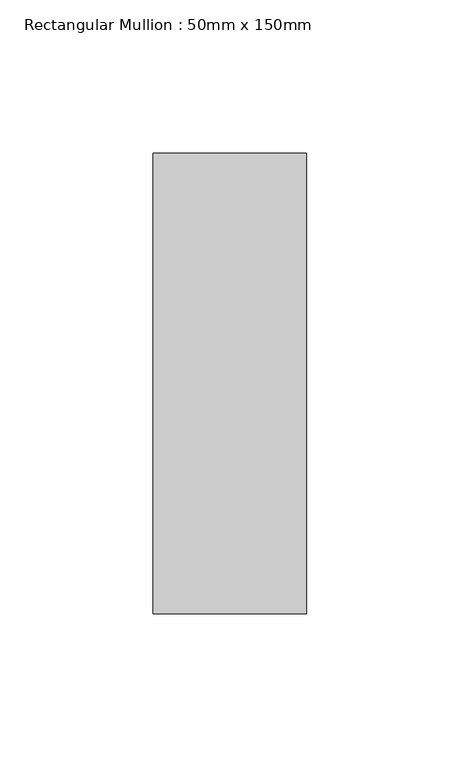
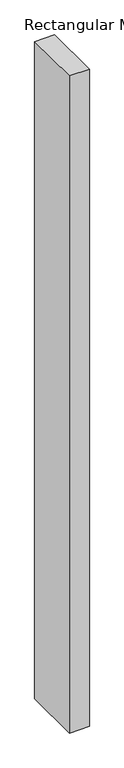
"""IFC4 building model written with IfcOpenShell, lengths in millimetres: member geometry, Rectangular Mullion : 50mm x 150mm."""

import ifcopenshell
import ifcopenshell.guid

model = None  # the IFC model being written
_history = None  # IfcOwnerHistory: only IFC2X3 demands one
_inside = {}  # id of a spatial element -> (the spatial element, [elements in it])
_under = {}  # id of a project, library or spatial element -> (it, [spatial elements below it])
_declared = {}  # id of a project -> (the project, [libraries it declares])
_typed = {}  # id of a type object -> (the type object, [elements of that type])
_made_of = {}  # id of a material, layer set ... -> (it, [elements and type objects made of it])


def new_model(schema):
    """Start an empty IFC model of exactly this schema.

    Asked for "IFC4X3", IfcOpenShell would pick the latest addendum, in which some entities
    have other attributes; the version numbers below select the first issue.
    IFC2X3 requires an IfcOwnerHistory on every rooted entity: one is made here for all.
    """
    global model, _history
    if schema == "IFC4X3":
        model = ifcopenshell.file(schema_version=(4, 3, 0, 0))
    else:
        model = ifcopenshell.file(schema=schema)
    _inside.clear()
    _under.clear()
    _declared.clear()
    _typed.clear()
    _made_of.clear()
    _history = None
    if model.schema == "IFC2X3":
        org = make("IfcOrganization", Name="unknown")
        user = make(
            "IfcPersonAndOrganization",
            ThePerson=make("IfcPerson", FamilyName="unknown"),
            TheOrganization=org,
        )
        app = make(
            "IfcApplication",
            ApplicationDeveloper=org,
            Version="unknown",
            ApplicationFullName="unknown",
            ApplicationIdentifier="unknown",
        )
        _history = make(
            "IfcOwnerHistory",
            OwningUser=user,
            OwningApplication=app,
            ChangeAction="ADDED",
            CreationDate=0,
        )
    return model


def make(cls, **values):
    """One entity of the class cls with the attributes given. An attribute that is None is left unset."""
    return model.create_entity(
        cls, **{name: value for name, value in values.items() if value is not None}
    )


def rooted(cls, **values):
    """An entity with a GlobalId (a new one), such as an element, a storey or a relation."""
    return make(cls, GlobalId=ifcopenshell.guid.new(), OwnerHistory=_history, **values)


def si_unit(unit_type, name, prefix=None):
    """IfcSIUnit, for example si_unit("LENGTHUNIT", "METRE", prefix="MILLI")."""
    return make("IfcSIUnit", UnitType=unit_type, Prefix=prefix, Name=name)


def assignment(units):
    """IfcUnitAssignment: the units of a project."""
    return None if units is None else make("IfcUnitAssignment", Units=units)


def point(xyz):
    """IfcCartesianPoint."""
    return None if xyz is None else make("IfcCartesianPoint", Coordinates=xyz)


def direction(xyz):
    """IfcDirection."""
    return None if xyz is None else make("IfcDirection", DirectionRatios=xyz)


def frame(location, z_axis=None, x_axis=None):
    """IfcAxis2Placement3D, a coordinate frame: its origin and axes. An axis left out is left unset."""
    return make(
        "IfcAxis2Placement3D",
        Location=point(location),
        Axis=direction(z_axis),
        RefDirection=direction(x_axis),
    )


def origin():
    """The frame at (0, 0, 0) with its axes left unset."""
    return frame((0.0, 0.0, 0.0))


def place(relative_to, where):
    """IfcLocalPlacement: puts the frame where relative to a parent placement (None: the world)."""
    return make(
        "IfcLocalPlacement", PlacementRelTo=relative_to, RelativePlacement=where
    )


def context(
    kind, dimensions, precision=None, world=None, true_north=None, identifier=None
):
    """IfcGeometricRepresentationContext, for example the 3D "Model" context."""
    return make(
        "IfcGeometricRepresentationContext",
        ContextIdentifier=identifier,
        ContextType=kind,
        CoordinateSpaceDimension=dimensions,
        Precision=precision,
        WorldCoordinateSystem=world,
        TrueNorth=true_north,
    )


def project(units=None, contexts=None):
    """IfcProject with its units and contexts."""
    return rooted(
        "IfcProject",
        Name="project",
        RepresentationContexts=contexts,
        UnitsInContext=assignment(units),
    )


def spatial(cls, under=None, at=None, **own):
    """A site, building, storey or space (cls), placed at a placement, below another one or the project."""
    s = rooted(cls, ObjectPlacement=at, **own)
    if under is not None:
        _under.setdefault(under.id(), (under, []))[1].append(s)
    return s


def polyline(points):
    """IfcPolyline through the points."""
    return make("IfcPolyline", Points=[point(p) for p in points])


def outline(outer, holes=None, kind="AREA"):
    """IfcArbitraryClosedProfileDef: a profile drawn as a closed curve; with holes, ...WithVoids."""
    if holes is None:
        return make("IfcArbitraryClosedProfileDef", ProfileType=kind, OuterCurve=outer)
    return make(
        "IfcArbitraryProfileDefWithVoids",
        ProfileType=kind,
        OuterCurve=outer,
        InnerCurves=holes,
    )


def extrude(swept, where, along, depth):
    """IfcExtrudedAreaSolid: the profile swept, set in the frame where, extruded along a direction by depth."""
    return make(
        "IfcExtrudedAreaSolid",
        SweptArea=swept,
        Position=where,
        ExtrudedDirection=direction(along),
        Depth=depth,
    )


def shape(context_of_items, identifier, shape_type, items):
    """IfcShapeRepresentation: the items that make up one representation, for example the "Body"."""
    return make(
        "IfcShapeRepresentation",
        ContextOfItems=context_of_items,
        RepresentationIdentifier=identifier,
        RepresentationType=shape_type,
        Items=items,
    )


def source(mapping_origin, context_of_items, identifier, shape_type, items):
    """IfcRepresentationMap: a shape defined once, which mapped items show again and again."""
    return make(
        "IfcRepresentationMap",
        MappingOrigin=mapping_origin,
        MappedRepresentation=shape(context_of_items, identifier, shape_type, items),
    )


def transform(
    local_origin,
    x_axis=None,
    y_axis=None,
    z_axis=None,
    scale=None,
    scale2=None,
    scale3=None,
    uniform=True,
):
    """IfcCartesianTransformationOperator3D, or its non-uniform kind. x_axis, y_axis, z_axis: its Axis1, 2, 3."""
    if uniform:
        return make(
            "IfcCartesianTransformationOperator3D",
            Axis1=direction(x_axis),
            Axis2=direction(y_axis),
            LocalOrigin=point(local_origin),
            Scale=scale,
            Axis3=direction(z_axis),
        )
    return make(
        "IfcCartesianTransformationOperator3DnonUniform",
        Axis1=direction(x_axis),
        Axis2=direction(y_axis),
        LocalOrigin=point(local_origin),
        Scale=scale,
        Axis3=direction(z_axis),
        Scale2=scale2,
        Scale3=scale3,
    )


def mapped(mapping_source, mapping_target):
    """IfcMappedItem: shows the shape of a source again, moved by a transform."""
    return make(
        "IfcMappedItem", MappingSource=mapping_source, MappingTarget=mapping_target
    )


def made_of(thing, what):
    """Note that an element or type object is made of a material, layer set ...; save() writes the relation."""
    if what is not None:
        _made_of.setdefault(what.id(), (what, []))[1].append(thing)
    return thing


def element(
    cls,
    number,
    at=None,
    inside=None,
    cuts=None,
    type_object=None,
    material=None,
    context=None,
    identifier="Body",
    shape_type=None,
    held_by="IfcProductDefinitionShape",
    body=None,
    shapes=None,
    **own,
):
    """One element of the class cls, such as IfcWall. Its Tag is "e" and its number.

    at: its placement. inside: the storey or other place that contains it. cuts: it is an
    opening in that element (IfcRelVoidsElement). A single representation is given by context,
    identifier, shape_type and body (its items); several are given by shapes. held_by: the class
    of the entity that holds the representations. save() writes the other relations.
    """
    e = rooted(cls, Tag="e%d" % number, ObjectPlacement=at, **own)
    if body is not None:
        shapes = [shape(context, identifier, shape_type, body)]
    if shapes is not None:
        e.Representation = make(held_by, Representations=shapes)
    if inside is not None:
        _inside.setdefault(inside.id(), (inside, []))[1].append(e)
    if cuts is not None:
        rooted(
            "IfcRelVoidsElement", RelatingBuildingElement=cuts, RelatedOpeningElement=e
        )
    if type_object is not None:
        _typed.setdefault(type_object.id(), (type_object, []))[1].append(e)
    return made_of(e, material)


def aggregate(whole, parts):
    """IfcRelAggregates: a whole, such as a stair, and the parts it consists of."""
    return rooted("IfcRelAggregates", RelatingObject=whole, RelatedObjects=parts)


def save(model, path):
    """Write the relations noted so far, then the file.

    IfcRelAggregates (storeys below a building ...), IfcRelContainedInSpatialStructure (elements
    in a storey), IfcRelDefinesByType, IfcRelAssociatesMaterial and IfcRelDeclares: one each for
    every whole, place, type object, material and project.
    """
    for whole, parts in _under.values():
        aggregate(whole, parts)
    for where, things in _inside.values():
        rooted(
            "IfcRelContainedInSpatialStructure",
            RelatedElements=things,
            RelatingStructure=where,
        )
    for kind, things in _typed.values():
        rooted("IfcRelDefinesByType", RelatedObjects=things, RelatingType=kind)
    for what, things in _made_of.values():
        rooted("IfcRelAssociatesMaterial", RelatedObjects=things, RelatingMaterial=what)
    for by, libraries in _declared.values():
        rooted("IfcRelDeclares", RelatingContext=by, RelatedDefinitions=libraries)
    model.write(path)


def rectangular_mullion_50mm_x_150mm_0deb6731(model_context):
    return source(origin(), model_context, "Body", "SweptSolid", [
        extrude(outline(polyline([(0.0, 75.0), (0.0, -75.0), (-50.0, -75.0), (-50.0, 75.0), (0.0, 75.0)])), frame((0.0, 0.0, -1736.2355347), z_axis=(0.0, 0.0, 1.0), x_axis=(1.0, 0.0, 0.0)), (0.0, 0.0, 1.0), 1736.2355347),
    ])


if __name__ == "__main__":
    model = new_model("IFC4")
    model_context = context("Model", 3, world=origin())
    ifc_project = project(units=[si_unit("LENGTHUNIT", "METRE", prefix="MILLI")], contexts=[model_context])
    site = spatial("IfcSite", under=ifc_project)
    building = spatial("IfcBuilding", under=site)
    placement = place(None, origin())
    rectangular_mullion_50mm_x_150mm_shape = rectangular_mullion_50mm_x_150mm_0deb6731(model_context)
    element("IfcMember", 1, ObjectType="Rectangular Mullion : 50mm x 150mm", at=placement, inside=building, context=model_context, shape_type="MappedRepresentation", body=[
        mapped(rectangular_mullion_50mm_x_150mm_shape, transform((0.0, 0.0, 0.0), x_axis=(1.0, 0.0, 0.0), y_axis=(0.0, 1.0, 0.0), z_axis=(0.0, 0.0, 1.0))),
    ])
    save(model, "model.ifc")

# Revit data of these elements
# Type "Rectangular Mullion : 50mm x 150mm"
#   built-in parameter 1007304 = 0.492126 (stored number, unit not read)
#   built-in parameter 1007301 = 0.082021 (stored number, unit not read)
#   built-in parameter 1007300 = 0.082021 (stored number, unit not read)
# Element 1 (IfcMember, "Rectangular Mullion : 50mm x 150mm")
#   Materials on its faces: "Aluminum"
# Materials
#   "Aluminum": class "Metal", colour RGB 244 244 244, transparency 0, Description = "Aluminum 6061", Cost = 0
